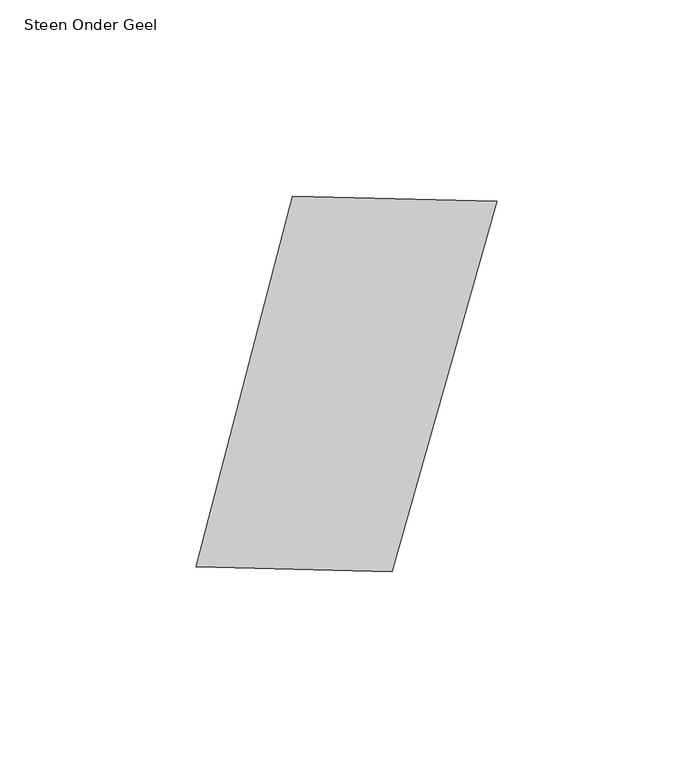
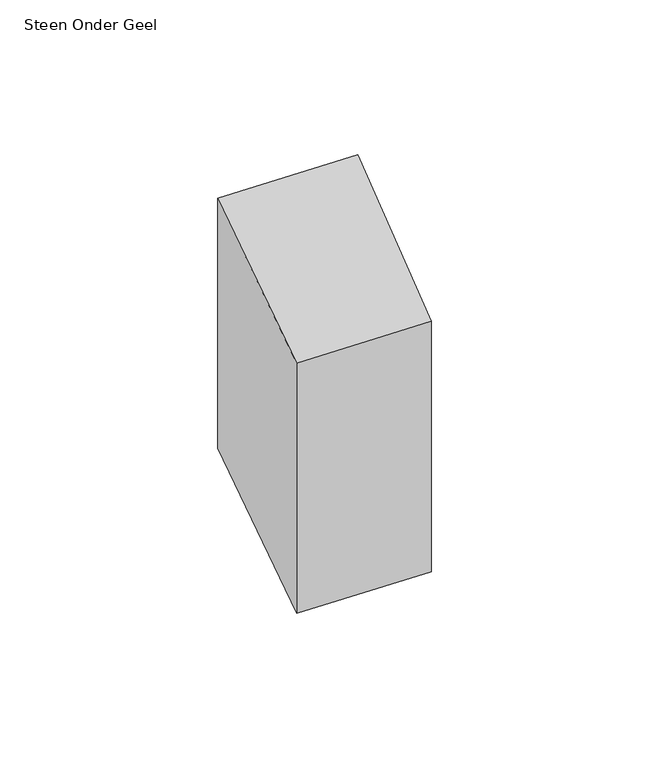
"""IFC4 building model written with IfcOpenShell, lengths in millimetres: proxy geometry, 00_GMA_steen_versie_4 : Steen Onder Geel."""

from ifc_helpers import new_model, si_unit, origin, origin_with_axes, place, context, project, spatial, polyline, outline, extrude, source, transform, mapped, element, save


def steen_onder_geel_8b684e23(model_context):
    return source(origin(), model_context, "Body", "SweptSolid", [
        extrude(outline(polyline([(113.250011, 113.5671988), (86.4975414, 19.0691956), (36.5140223, 20.3528666), (61.1462748, 114.8844291), (113.250011, 113.5671988)])), origin_with_axes(), (0.0, 0.0, 1.0), 100.0),
    ])


if __name__ == "__main__":
    model = new_model("IFC4")
    model_context = context("Model", 3, world=origin())
    ifc_project = project(units=[si_unit("LENGTHUNIT", "METRE", prefix="MILLI")], contexts=[model_context])
    site = spatial("IfcSite", under=ifc_project)
    building = spatial("IfcBuilding", under=site)
    placement = place(None, origin())
    steen_onder_geel_shape = steen_onder_geel_8b684e23(model_context)
    element("IfcBuildingElementProxy", 1, Name="00_GMA_steen_versie_4 : Steen Onder Geel", ObjectType="00_GMA_steen_versie_4 : Steen Onder Geel", at=placement, inside=building, context=model_context, shape_type="MappedRepresentation", body=[
        mapped(steen_onder_geel_shape, transform((0.0, 0.0, 0.0), x_axis=(1.0, 0.0, 0.0), y_axis=(0.0, 1.0, 0.0), z_axis=(0.0, 0.0, 1.0))),
    ])
    save(model, "model.ifc")

# Revit data of these elements
# Type "00_GMA_steen_versie_4 : Steen Onder Geel"
#   StootVoegHalfBoven [instance default] = 5 mm
#   StootVoegHalf [instance default] = 5 mm
#   StootVoegBreedteOnder = 10 mm
#   StootVoegBreedteBoven = 10 mm
#   Steendikte = 100 mm
#   LintVoegOnderHalf = 0 mm
#   LintVoegOnder = 0 mm
#   LintVoegBovenHalf = 5 mm
#   LintVoegBoven = 10 mm
#   materiaal = 21_steen_geel
#   MateriaalVoeg = none
#   Default Elevation = 0
# Element 1 (IfcBuildingElementProxy, "00_GMA_steen_versie_4 : Steen Onder Geel")
#   Materials on its faces: "21_steen_geel"
# Materials
#   "21_steen_geel": class "Unassigned", colour RGB 202 202 0, transparency 0, Cost = 0
